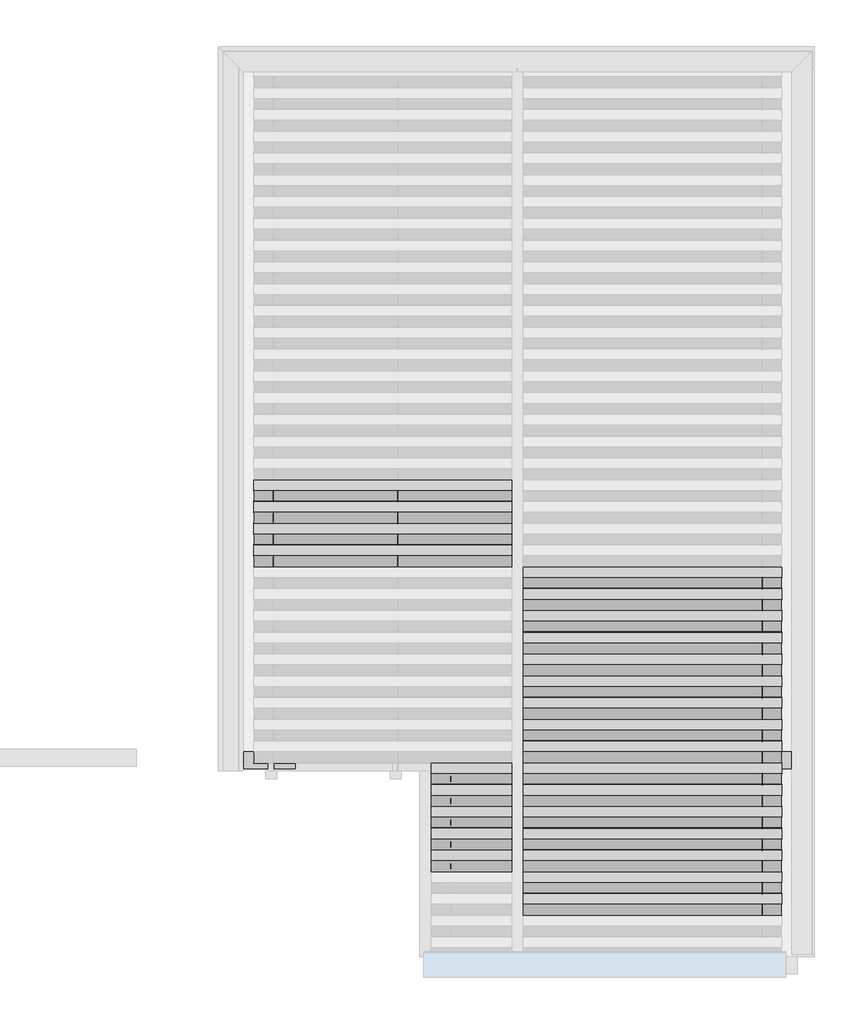
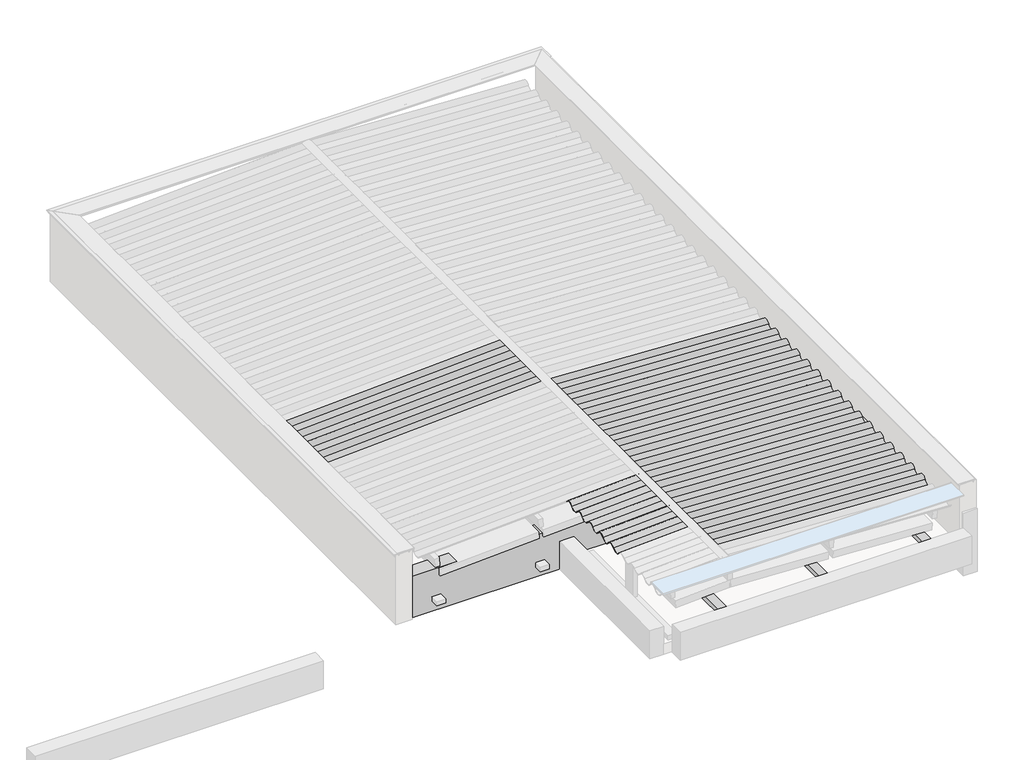
# One storey, part 2 of 4: 34 beams, 7 columns.
# Revit data of these elements (continued)
# Element 9 (IfcBeam, "TQS - Viga retangular : 19.0 x 60.0") (continued)
#   Largura gerber direita = 0.00 m
#   Resultado de Ensaios fck (MPa) = 0
#   Unique TQS ID = -345
#   Principal = yes
#   Structural Material = none
#   Phase Created = CC_PE
# Elements 10, 11, 12, 13, 14, 15, 16, 17, 18, 19, 20, 21, 22, 23, 24, 25, 26, 27, 28, 29, 30, 31, 32, 33, 34 (IfcBeam, "Telha Ondulada : Fibrocimento")
#   Phase Created = CC_PE
#   Materials on its faces: ".TELHA DE FIBROCIMENTO"
# Elements 35, 36, 37, 38, 39, 40, 41 (IfcColumn, "Madeira de lei-Coluna : Pontalete 6X16cm")
#   Comments = ""
#   Structural Material = .MADEIRAMENTO
#   Phase Created = CC_PE
#   Materials on its faces: ".MADEIRAMENTO"
# Materials
#   ".TELHA DE FIBROCIMENTO": class "CC_TELHADO", colour RGB 77 77 76, transparency 0, Description = "TELHA ONDULADA FIBROCIMENTO", Cost = 0
#   ".MADEIRAMENTO": class ".CC_MADEIRAS", colour RGB 212 179 113, transparency 0, Cost = 0
